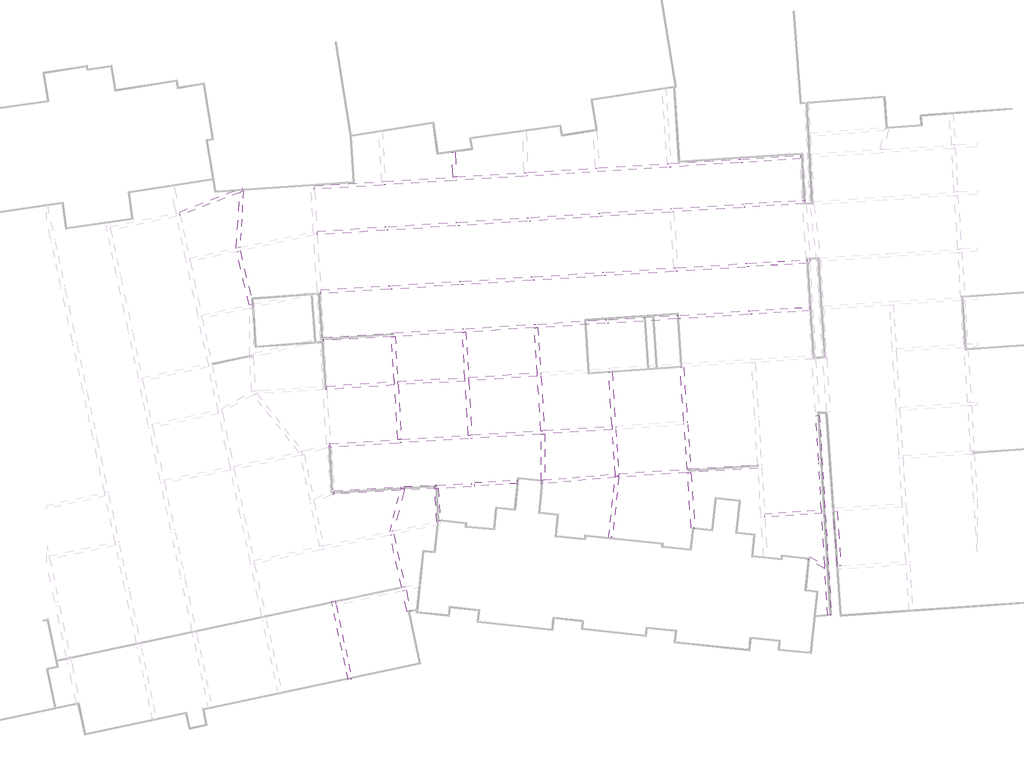
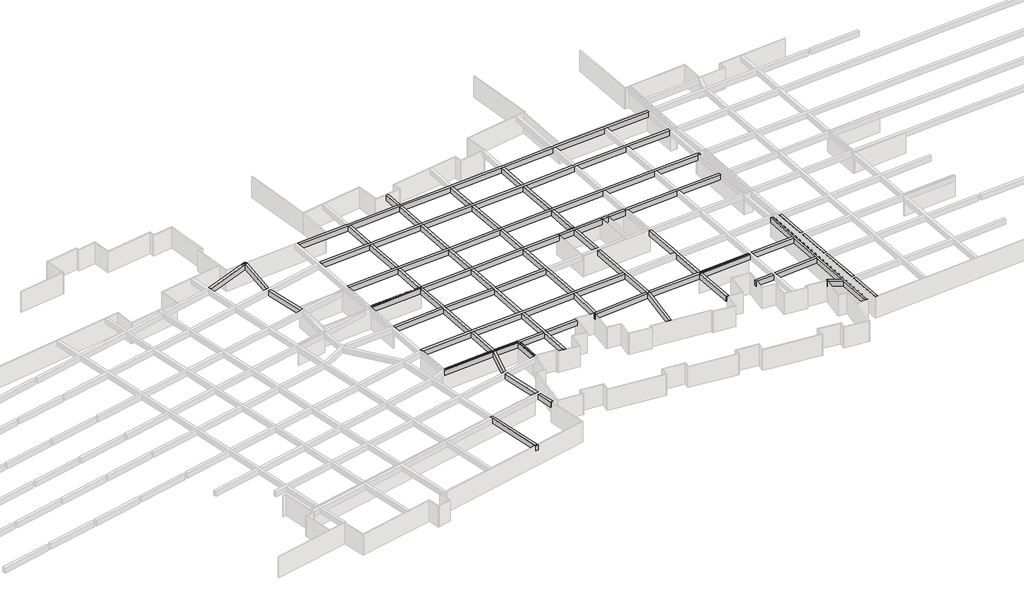
# One storey, part 11 of 14: 35 beams.
# Revit data of these elements (continued)
# Type "混凝土 - 矩形梁 : KL_beam" (continued)
#   Structural Material [instance default] = 混凝土 - 现场浇注混凝土
#   Assembly Code = ""
# Elements 1, 2, 3, 4, 5, 6, 7, 8, 9, 10, 11, 12, 13, 14, 15, 16, 17, 18, 19, 20, 21, 22, 23, 24, 25, 26, 27, 28, 29, 30, 31, 32, 33, 34, 35 (IfcBeam, "混凝土 - 矩形梁 : KL_beam")
#   Comments = ""
#   Structural Material = none
#   Phase Created = 新构造
# Materials
#   "混凝土 - 现场浇注混凝土": class "混凝土", colour RGB 192 192 192, transparency 0
